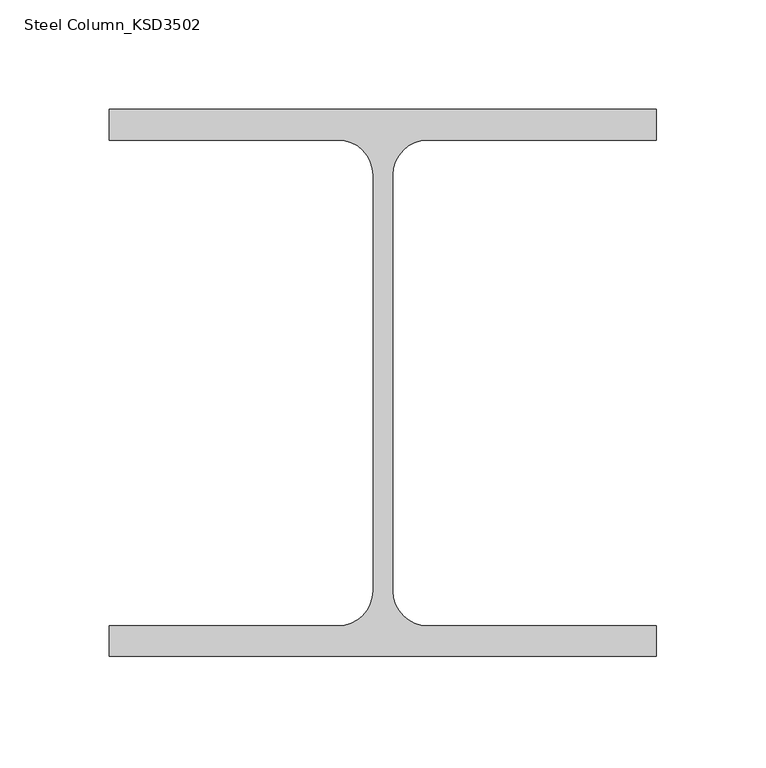
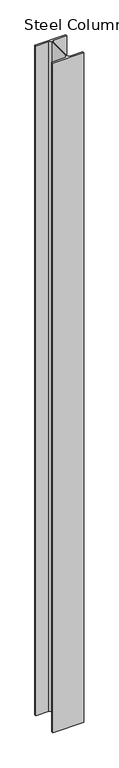
"""IFC4 building model written with IfcOpenShell, lengths in millimetres: column geometry, Steel Column_KSD3502 : H_SC_ASC_H-250×250x9x14."""

from ifc_helpers import new_model, si_unit, point, frame, frame_2d, origin, place, context, project, spatial, polyline, circle_curve, trimmed, segment, composite_curve, outline, extrude, source, transform, mapped, element, save


def steel_column_ksd3502_6a202524(model_context):
    return source(origin(), model_context, "Body", "SweptSolid", [
        extrude(outline(composite_curve([segment(polyline([(125.0, 125.0), (125.0, 111.0), (20.5, 111.0)]), True, "CONTINUOUS"), segment(trimmed(circle_curve(frame_2d((20.5, 95.0)), 16.0), [point((20.5, 111.0))], [point((4.5, 95.0))], True, "CARTESIAN"), True, "CONTINUOUS"), segment(polyline([(4.5, 95.0), (4.5, -95.0)]), True, "CONTINUOUS"), segment(trimmed(circle_curve(frame_2d((20.5, -95.0)), 16.0), [point((4.5, -95.0))], [point((20.5, -111.0))], True, "CARTESIAN"), True, "CONTINUOUS"), segment(polyline([(20.5, -111.0), (125.0, -111.0), (125.0, -125.0), (-125.0, -125.0), (-125.0, -111.0), (-20.5, -111.0)]), True, "CONTINUOUS"), segment(trimmed(circle_curve(frame_2d((-20.5, -95.0)), 16.0), [point((-20.5, -111.0))], [point((-4.5, -95.0))], True, "CARTESIAN"), True, "CONTINUOUS"), segment(polyline([(-4.5, -95.0), (-4.5, 95.0)]), True, "CONTINUOUS"), segment(trimmed(circle_curve(frame_2d((-20.5, 95.0)), 16.0), [point((-4.5, 95.0))], [point((-20.5, 111.0))], True, "CARTESIAN"), True, "CONTINUOUS"), segment(polyline([(-20.5, 111.0), (-125.0, 111.0), (-125.0, 125.0), (125.0, 125.0)]), True, "CONTINUOUS")], self_intersect=False)), frame((0.0, 0.0, 599.9720055), z_axis=(0.0, 0.0, 1.0), x_axis=(1.0, 0.0, 0.0)), (0.0, 0.0, 1.0), 5700.0),
    ])


if __name__ == "__main__":
    model = new_model("IFC4")
    model_context = context("Model", 3, world=origin())
    ifc_project = project(units=[si_unit("LENGTHUNIT", "METRE", prefix="MILLI")], contexts=[model_context])
    site = spatial("IfcSite", under=ifc_project)
    building = spatial("IfcBuilding", under=site)
    placement = place(None, origin())
    steel_column_ksd3502_shape = steel_column_ksd3502_6a202524(model_context)
    element("IfcColumn", 1, ObjectType="Steel Column_KSD3502 : H_SC_ASC_H-250×250x9x14", at=placement, inside=building, context=model_context, shape_type="MappedRepresentation", body=[
        mapped(steel_column_ksd3502_shape, transform((0.0, 0.0, 0.0), x_axis=(1.0, 0.0, 0.0), y_axis=(0.0, 1.0, 0.0), z_axis=(0.0, 0.0, 1.0))),
    ])
    save(model, "model.ifc")

# Revit data of these elements
# Type "Steel Column_KSD3502 : H_SC_ASC_H-250×250x9x14"
#   Width = 25.0 cm
#   Web Thickness = 0.9 cm
#   Web Fillet = 1.6 cm
#   Warping Constant = 507646.0 cm⁶
#   Torsional Moment of Inertia = 51.4681 cm⁴
#   Section Area = 92.18 cm²
#   Plastic Modulus weak axis = 444.0 cm³
#   Plastic Modulus strong axis = 960.0 cm³
#   Perimeter = 1.27 m²/m
#   Nominal Weight = 72.40 kgf/m
#   Moment of Inertia weak axis = 3650.00 cm⁴
#   Moment of Inertia strong axis = 10800.00 cm⁴
#   Height = 25.0 cm
#   Flange Thickness = 1.4 cm
#   Elastic Modulus weak axis = 292.0 cm³
#   Elastic Modulus strong axis = 867.0 cm³
#   Centroid Vertical = 12.5 cm
#   Centroid Horizontal = 12.5 cm
#   Bolt Spacing = 13.97 cm
#   Structural Material [instance default] = Steel, 45-345
#   Section Name Key = ""
#   Assembly Code = ""
# Element 1 (IfcColumn, "Steel Column_KSD3502 : H_SC_ASC_H-250×250x9x14")
#   Structural Material = A03AD029-00005_Anchor Bolt (Installation only)_M24
#   Materials on its faces: "A03AD029-00005_Anchor Bolt (Installation only)_M24"
# Materials
#   "Steel, 45-345": class "Metal", colour RGB 189 187 185, transparency 0, Description = "Steel 345 MPa", Cost = 0
#   "A03AD029-00005_Anchor Bolt (Installation only)_M24": class "Unassigned", colour RGB 84 83 81, transparency 0, Cost = 0
